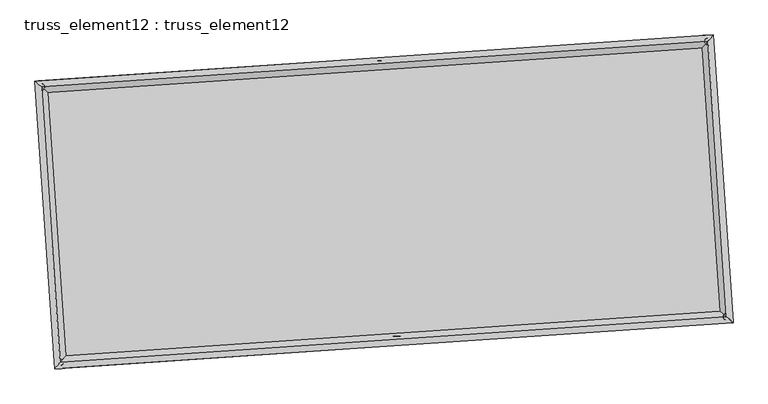
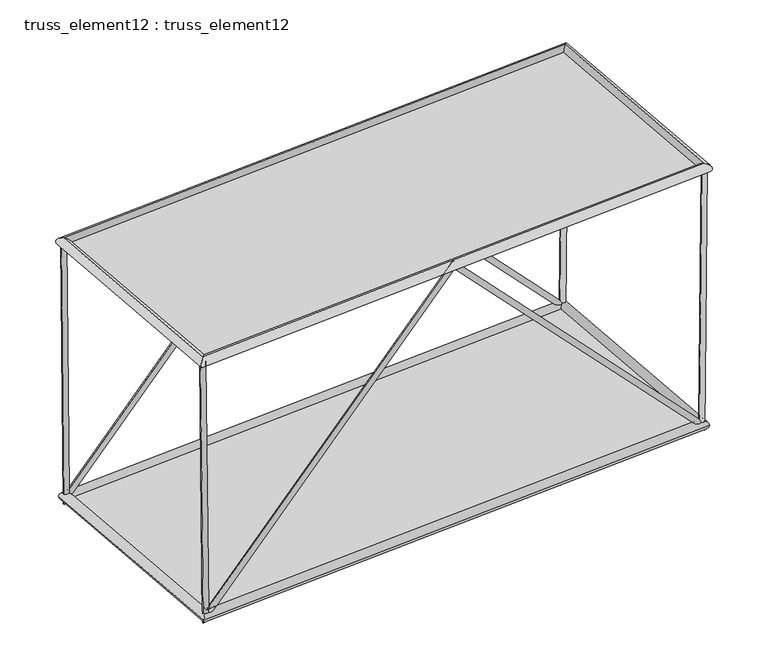
"""IFC4 building model written with IfcOpenShell, lengths in millimetres: plate geometry, truss_element12 : truss_element12."""

from ifc_helpers import new_model, si_unit, frame, origin, origin_with_axes, place, context, project, spatial, polyline, circle_curve, ellipse_curve, outline, extrude, source, transform, mapped, element, save
from ifc_brep_helpers import plane_surface, cylinder_surface, advanced_brep


def truss_element12_truss_element12_5452cb03(model_context):
    return source(origin(), model_context, "Body", "SolidModel", [
        advanced_brep(
        [(-3715.2018839, 2272.796917, 5000.248885), (-3814.3001969, 2259.4360138, 4999.2435881), (-3666.1746751, 2276.139896, 122.9048146), (-3762.8122077, 2262.9467841, -122.9048146), (1064.1683221, 2598.6840033, 5071.8637106), (1064.609821, 2592.1103415, 4927.6196838), (5793.6352732, 2921.1683763, 122.8985374), (5891.1257038, 2921.2121122, -122.8985374), (5843.5319155, 2924.5706386, 5000.2487185), (5943.5264514, 2924.78512, 4999.2255971)],
        [
            (0, 1, circle_curve(frame((-3764.7510404, 2266.1164654, 4999.7462366), z_axis=(-0.010051519791738989, -0.0006853749251947657, 0.9999492473176268), x_axis=(-0.1336091408985775, 0.991033882804214, -0.000663778839363479)), 50.0)),
            (1, 0, circle_curve(frame((-3764.7510404, 2266.1164654, 4999.7462366), z_axis=(-0.010051519791738989, -0.0006853749251947657, 0.9999492473176268), x_axis=(-0.1336091408985775, 0.991033882804214, -0.000663778839363479)), 50.0)),
            (0, 2),
            (2, 3, ellipse_curve(frame((-3714.4934414, 2269.54334, 0.0), z_axis=(-0.9276377400160163, -0.06325209121051249, 0.36808612613826514), x_axis=(0.3672334163736698, 0.025040250677613063, 0.9297916991157348)), 132.4731533, 50.0)),
            (3, 1),
            (3, 2, ellipse_curve(frame((-3714.4934414, 2269.54334, 0.0), z_axis=(-0.9276377400160163, -0.06325209121051249, 0.36808612613826514), x_axis=(0.3672334163736698, 0.025040250677613063, 0.9297916991157348)), 132.4731533, 50.0)),
            (2, 4),
            (4, 5, ellipse_curve(frame((1064.3890715, 2595.3971724, 4999.7416972), z_axis=(-0.9976833949926481, -0.06802823815490638, 4.657770887637942e-05), x_axis=(-4.6469806773262635e-05, -3.1685994756930008e-06, -0.9999999989152585)), 72.2790583, 50.0)),
            (5, 3),
            (5, 4, ellipse_curve(frame((1064.3890715, 2595.3971724, 4999.7416972), z_axis=(-0.9976833949926481, -0.06802823815490638, 4.657770887637942e-05), x_axis=(-4.6469806773262635e-05, -3.1685994756930008e-06, -0.9999999989152585)), 72.2790583, 50.0)),
            (4, 6),
            (6, 7, ellipse_curve(frame((5842.3804885, 2921.1902443, 0.0), z_axis=(-0.9276876380424469, -0.06325549356725449, -0.36795976513307666), x_axis=(-0.36710734809688195, -0.025031654561049187, 0.9298417130045366)), 132.4592623, 50.0)),
            (7, 5),
            (7, 6, ellipse_curve(frame((5842.3804885, 2921.1902443, 0.0), z_axis=(-0.9276876380424469, -0.06325549356725449, -0.36795976513307666), x_axis=(-0.36710734809688195, -0.025031654561049187, 0.9298417130045366)), 132.4592623, 50.0)),
            (8, 9, circle_curve(frame((5893.5291834, 2924.6778793, 4999.7371578), z_axis=(0.01022973898914847, 0.0006975270147915611, 0.9999474315664186), x_axis=(-0.0021518374254831385, 0.9999974566120504, -0.0006755480180010986)), 50.0)),
            (9, 8, circle_curve(frame((5893.5291834, 2924.6778793, 4999.7371578), z_axis=(0.01022973898914847, 0.0006975270147915611, 0.9999474315664186), x_axis=(-0.0021518374254831385, 0.9999974566120504, -0.0006755480180010986)), 50.0)),
            (6, 8),
            (9, 7),
        ],
        [
            plane_surface(frame((-3764.7510404, 2316.1164537, 4999.7805071), z_axis=(-0.010051519791740156, -0.0006853749251952957, 0.9999492473176268), x_axis=(0.9999494821989141, -6.889407663024368e-06, 0.010051517430706975))),
            cylinder_surface(frame((-3764.7510404, 2266.1164654, 4999.7462366), z_axis=(-0.010051519791738989, -0.0006853749251947657, 0.9999492473176268), x_axis=(-0.1336091408985775, 0.991033882804214, -0.000663778839363479)), 50.0),
            cylinder_surface(frame((-3714.4934414, 2269.54334, 0.0), z_axis=(-0.6901943166001666, -0.047061726774740055, -0.7220920988390671), x_axis=(-0.02041583735188898, 0.9987521038850324, -0.04557881712421584)), 50.0),
            cylinder_surface(frame((1064.3890715, 2595.3971724, 4999.7416972), z_axis=(-0.6901272026448988, -0.047057150529254216, 0.7221565403384463), x_axis=(-0.11534925749082463, 0.9922789548414734, -0.045574385075704216)), 50.0),
            plane_surface(frame((5893.5291834, 2874.6778915, 4999.772036), z_axis=(0.01022973898914786, 0.0006975270147901555, 0.9999474315664189), x_axis=(0.9999476748511464, -7.13589268563908e-06, -0.010229736500278365))),
            cylinder_surface(frame((5842.3804885, 2921.1902443, 0.0), z_axis=(-0.010229738989148472, -0.0006975270147915612, -0.9999474315664189), x_axis=(-0.0021518374254831385, 0.9999974566120504, -0.0006755480180010986)), 50.0),
        ],
        [
            (0, [[1, 2]]),
            (1, [[-1, 3, 4, 5]]),
            (1, [[-2, -5, 6, -3]]),
            (2, [[-4, 7, 8, 9]]),
            (2, [[-6, -9, 10, -7]]),
            (3, [[-8, 11, 12, 13]]),
            (3, [[-10, -13, 14, -11]]),
            (4, [[15, 16]]),
            (5, [[-12, 17, -16, 18]]),
            (5, [[-14, -18, -15, -17]]),
        ],
    ),
        advanced_brep(
        [(-3443.0889309, -1717.9366673, 5000.248885), (-3542.187244, -1731.2975705, 4999.2435881), (-3394.0617222, -1714.5936883, 122.9048146), (-3490.6992548, -1727.7868002, -122.9048146), (1336.281275, -1392.049581, 5071.8637106), (1336.7227739, -1398.6232428, 4927.6196838), (6065.7482261, -1069.565208, 122.8985374), (6163.2386567, -1069.5214721, -122.8985374), (6115.6448684, -1066.1629457, 5000.2487185), (6215.6394043, -1065.9484643, 4999.2255971)],
        [
            (0, 1, circle_curve(frame((-3492.6380875, -1724.6171189, 4999.7462366), z_axis=(-0.010051519791739193, -0.000685374925194784, 0.9999492473176267), x_axis=(-0.13360914089857726, 0.991033882804214, -0.0006637788393634854)), 50.0)),
            (1, 0, circle_curve(frame((-3492.6380875, -1724.6171189, 4999.7462366), z_axis=(-0.010051519791739193, -0.000685374925194784, 0.9999492473176267), x_axis=(-0.13360914089857726, 0.991033882804214, -0.0006637788393634854)), 50.0)),
            (0, 2),
            (2, 3, ellipse_curve(frame((-3442.3804885, -1721.1902443, 0.0), z_axis=(-0.9276377400160165, -0.06325209121051241, 0.3680861261382646), x_axis=(0.36723341637366924, 0.025040250677612983, 0.929791699115735)), 132.4731533, 50.0)),
            (3, 1),
            (3, 2, ellipse_curve(frame((-3442.3804885, -1721.1902443, 0.0), z_axis=(-0.9276377400160165, -0.06325209121051241, 0.3680861261382646), x_axis=(0.36723341637366924, 0.025040250677612983, 0.929791699115735)), 132.4731533, 50.0)),
            (2, 4),
            (4, 5, ellipse_curve(frame((1336.5020245, -1395.3364119, 4999.7416972), z_axis=(-0.9976833949926481, -0.0680282381549063, 4.657770887573745e-05), x_axis=(-4.646980677264766e-05, -3.168599475625738e-06, -0.9999999989152585)), 72.2790583, 50.0)),
            (5, 3),
            (5, 4, ellipse_curve(frame((1336.5020245, -1395.3364119, 4999.7416972), z_axis=(-0.9976833949926481, -0.0680282381549063, 4.657770887573745e-05), x_axis=(-4.646980677264766e-05, -3.168599475625738e-06, -0.9999999989152585)), 72.2790583, 50.0)),
            (4, 6),
            (6, 7, ellipse_curve(frame((6114.4934414, -1069.54334, 0.0), z_axis=(-0.9276876380424468, -0.06325549356725439, -0.36795976513307704), x_axis=(-0.3671073480968823, -0.025031654561049214, 0.9298417130045364)), 132.4592623, 50.0)),
            (7, 5),
            (7, 6, ellipse_curve(frame((6114.4934414, -1069.54334, 0.0), z_axis=(-0.9276876380424468, -0.06325549356725439, -0.36795976513307704), x_axis=(-0.3671073480968823, -0.025031654561049214, 0.9298417130045364)), 132.4592623, 50.0)),
            (8, 9, circle_curve(frame((6165.6421364, -1066.055705, 4999.7371578), z_axis=(0.010229738989148298, 0.0006975270147915052, 0.9999474315664186), x_axis=(-0.0021518374254831524, 0.9999974566120505, -0.0006755480180010431)), 50.0)),
            (9, 8, circle_curve(frame((6165.6421364, -1066.055705, 4999.7371578), z_axis=(0.010229738989148298, 0.0006975270147915052, 0.9999474315664186), x_axis=(-0.0021518374254831524, 0.9999974566120505, -0.0006755480180010431)), 50.0)),
            (6, 8),
            (9, 7),
        ],
        [
            plane_surface(frame((-3492.6380875, -1674.6171306, 4999.7805071), z_axis=(-0.010051519791740156, -0.0006853749251952938, 0.9999492473176268), x_axis=(0.9999494821989141, -6.889407663024368e-06, 0.010051517430706975))),
            cylinder_surface(frame((-3492.6380875, -1724.6171189, 4999.7462366), z_axis=(-0.010051519791739195, -0.0006853749251947842, 0.9999492473176269), x_axis=(-0.13360914089857726, 0.991033882804214, -0.0006637788393634854)), 50.0),
            cylinder_surface(frame((-3442.3804885, -1721.1902443, 0.0), z_axis=(-0.6901943166001662, -0.04706172677473995, -0.7220920988390676), x_axis=(-0.020415837351888903, 0.9987521038850324, -0.04557881712421575)), 50.0),
            cylinder_surface(frame((1336.5020245, -1395.3364119, 4999.7416972), z_axis=(-0.6901272026448991, -0.0470571505292542, 0.7221565403384458), x_axis=(-0.11534925749082446, 0.9922789548414734, -0.04557438507570417)), 50.0),
            plane_surface(frame((6165.6421364, -1116.0556928, 4999.772036), z_axis=(0.01022973898914786, 0.0006975270147901537, 0.9999474315664189), x_axis=(0.9999476748511464, -7.13589268563908e-06, -0.010229736500278365))),
            cylinder_surface(frame((6114.4934414, -1069.54334, 0.0), z_axis=(-0.0102297389891483, -0.0006975270147915053, -0.9999474315664189), x_axis=(-0.0021518374254831524, 0.9999974566120505, -0.0006755480180010431)), 50.0),
        ],
        [
            (0, [[1, 2]]),
            (1, [[-1, 3, 4, 5]]),
            (1, [[-2, -5, 6, -3]]),
            (2, [[-4, 7, 8, 9]]),
            (2, [[-6, -9, 10, -7]]),
            (3, [[-8, 11, 12, 13]]),
            (3, [[-10, -13, 14, -11]]),
            (4, [[15, 16]]),
            (5, [[-12, 17, -16, 18]]),
            (5, [[-14, -18, -15, -17]]),
        ],
    ),
        advanced_brep(
        [(-3492.6404759, -1724.619766, 4909.7462366), (-3492.635699, -1724.6144717, 5089.7462366), (-3764.7483147, 2266.114167, 5089.7462366), (-3764.753766, 2266.1187639, 4909.7462366), (5893.5269635, 2924.6752436, 5089.7371578), (5893.5314034, 2924.680515, 4909.7371579), (6165.6395791, -1066.053395, 5089.7371578), (6165.6446936, -1066.0580149, 4909.7371579)],
        [
            (0, 1, ellipse_curve(frame((-3492.6380875, -1724.6171189, 4999.7462366), z_axis=(-0.7535719234051445, 0.6573654662781055, 6.63138572682771e-07), x_axis=(-0.657365466277774, -0.7535719234054339, 6.631385726828099e-07)), 127.2792206, 90.0)),
            (1, 2),
            (2, 3, ellipse_curve(frame((-3764.7510404, 2266.1164654, 4999.7462366), z_axis=(-0.6573654662777743, -0.7535719234054338, 6.631385726828458e-07), x_axis=(0.7535719234051448, -0.6573654662781053, -6.631385726828071e-07)), 127.2792206, 90.0)),
            (3, 0),
            (1, 0, ellipse_curve(frame((-3492.6380875, -1724.6171189, 4999.7462366), z_axis=(-0.7535719234051445, 0.6573654662781055, 6.63138572682771e-07), x_axis=(-0.657365466277774, -0.7535719234054339, 6.631385726828099e-07)), 127.2792206, 90.0)),
            (3, 2, ellipse_curve(frame((-3764.7510404, 2266.1164654, 4999.7462366), z_axis=(-0.6573654662777743, -0.7535719234054338, 6.631385726828458e-07), x_axis=(0.7535719234051448, -0.6573654662781053, -6.631385726828071e-07)), 127.2792206, 90.0)),
            (2, 4),
            (4, 5, ellipse_curve(frame((5893.5291834, 2924.6778793, 4999.7371578), z_axis=(-0.7535719234051445, 0.6573654662781058, 6.63138572682843e-07), x_axis=(-0.6573654662777743, -0.7535719234054337, 6.631385726828096e-07)), 127.2792206, 90.0)),
            (5, 3),
            (5, 4, ellipse_curve(frame((5893.5291834, 2924.6778793, 4999.7371578), z_axis=(-0.7535719234051445, 0.6573654662781058, 6.63138572682843e-07), x_axis=(-0.6573654662777743, -0.7535719234054337, 6.631385726828096e-07)), 127.2792206, 90.0)),
            (4, 6),
            (6, 7, ellipse_curve(frame((6165.6421364, -1066.055705, 4999.7371578), z_axis=(0.6573654662777743, 0.7535719234054338, -6.631385726827738e-07), x_axis=(-0.7535719234051447, 0.6573654662781053, 6.631385726828074e-07)), 127.2792206, 90.0)),
            (7, 5),
            (7, 6, ellipse_curve(frame((6165.6421364, -1066.055705, 4999.7371578), z_axis=(0.6573654662777743, 0.7535719234054338, -6.631385726827738e-07), x_axis=(-0.7535719234051447, 0.6573654662781053, 6.631385726828074e-07)), 127.2792206, 90.0)),
            (6, 1),
            (0, 7),
        ],
        [
            cylinder_surface(frame((-3492.6380875, -1724.6171189, 4999.7462366), z_axis=(0.06802823822869596, -0.997683396074877, 0.0), x_axis=(-0.9976833956703363, -0.06802823820111187, 2.847736223492992e-05)), 90.0),
            cylinder_surface(frame((-3764.7510404, 2266.1164654, 4999.7462366), z_axis=(-0.9976833960744381, -0.06802823822866694, 9.378195632207894e-07), x_axis=(-0.06802823817713236, 0.9976833956982991, 2.753954267206479e-05)), 90.0),
            cylinder_surface(frame((5893.5291834, 2924.6778793, 4999.7371578), z_axis=(-0.06802823822869598, 0.9976833960748771, 0.0), x_axis=(0.9976833957218709, 0.06802823820462583, 2.6601723109199666e-05)), 90.0),
            cylinder_surface(frame((6165.6421364, -1066.055705, 4999.7371578), z_axis=(0.9976833960744381, 0.06802823822866695, -9.378195632207388e-07), x_axis=(0.06802823822866695, -0.9976833956947851, 2.75395426720648e-05)), 90.0),
        ],
        [
            (0, [[1, 2, 3, 4]]),
            (0, [[5, -4, 6, -2]]),
            (1, [[-3, 7, 8, 9]]),
            (1, [[-6, -9, 10, -7]]),
            (2, [[-8, 11, 12, 13]]),
            (2, [[-10, -13, 14, -11]]),
            (3, [[-12, 15, -1, 16]]),
            (3, [[-14, -16, -5, -15]]),
        ],
    ),
        advanced_brep(
        [(-3358.7115243, -1625.2761972, 0.0), (-3526.0494527, -1817.1042913, 0.0), (-3810.4074885, 2353.2123043, 0.0), (-3618.5793943, 2185.8743758, 0.0), (5926.0494527, 3017.1042913, 0.0), (5758.7115243, 2825.2761972, 0.0), (6210.4074885, -1153.2123043, 0.0), (6018.5793943, -985.8743758, 0.0)],
        [
            (0, 1, ellipse_curve(frame((-3442.3804885, -1721.1902443, 0.0), z_axis=(-0.7535719234054564, 0.6573654662780827, 0.0), x_axis=(-0.6573654662780827, -0.7535719234054563, 0.0)), 127.2792206, 90.0)),
            (1, 2),
            (2, 3, ellipse_curve(frame((-3714.4934414, 2269.54334, 0.0), z_axis=(-0.6573654662780827, -0.7535719234054565, 0.0), x_axis=(0.7535719234054565, -0.6573654662780822, 0.0)), 127.2792206, 90.0)),
            (3, 0),
            (1, 0, ellipse_curve(frame((-3442.3804885, -1721.1902443, 0.0), z_axis=(-0.7535719234054564, 0.6573654662780827, 0.0), x_axis=(-0.6573654662780827, -0.7535719234054563, 0.0)), 127.2792206, 90.0)),
            (3, 2, ellipse_curve(frame((-3714.4934414, 2269.54334, 0.0), z_axis=(-0.6573654662780827, -0.7535719234054565, 0.0), x_axis=(0.7535719234054565, -0.6573654662780822, 0.0)), 127.2792206, 90.0)),
            (2, 4),
            (4, 5, ellipse_curve(frame((5842.3804885, 2921.1902443, 0.0), z_axis=(-0.7535719234054563, 0.6573654662780826, 0.0), x_axis=(-0.6573654662780828, -0.7535719234054562, 0.0)), 127.2792206, 90.0)),
            (5, 3),
            (5, 4, ellipse_curve(frame((5842.3804885, 2921.1902443, 0.0), z_axis=(-0.7535719234054563, 0.6573654662780826, 0.0), x_axis=(-0.6573654662780828, -0.7535719234054562, 0.0)), 127.2792206, 90.0)),
            (4, 6),
            (6, 7, ellipse_curve(frame((6114.4934414, -1069.54334, 0.0), z_axis=(0.6573654662780825, 0.7535719234054565, 0.0), x_axis=(-0.7535719234054565, 0.6573654662780823, 0.0)), 127.2792206, 90.0)),
            (7, 5),
            (7, 6, ellipse_curve(frame((6114.4934414, -1069.54334, 0.0), z_axis=(0.6573654662780825, 0.7535719234054565, 0.0), x_axis=(-0.7535719234054565, 0.6573654662780823, 0.0)), 127.2792206, 90.0)),
            (6, 1),
            (0, 7),
        ],
        [
            cylinder_surface(frame((-3442.3804885, -1721.1902443, 0.0), z_axis=(0.06802823822869844, -0.9976833960748768, 0.0), x_axis=(-0.9976833960748768, -0.06802823822869844, 0.0)), 90.0),
            cylinder_surface(frame((-3714.4934414, 2269.54334, 0.0), z_axis=(-0.9976833960748768, -0.06802823822869929, 0.0), x_axis=(-0.06802823822869929, 0.9976833960748768, 0.0)), 90.0),
            cylinder_surface(frame((5842.3804885, 2921.1902443, 0.0), z_axis=(-0.06802823822869851, 0.9976833960748768, 0.0), x_axis=(0.9976833960748768, 0.06802823822869851, 0.0)), 90.0),
            cylinder_surface(frame((6114.4934414, -1069.54334, 0.0), z_axis=(0.9976833960748768, 0.06802823822869936, 0.0), x_axis=(0.06802823822869936, -0.9976833960748768, 0.0)), 90.0),
        ],
        [
            (0, [[1, 2, 3, 4]]),
            (0, [[5, -4, 6, -2]]),
            (1, [[-3, 7, 8, 9]]),
            (1, [[-6, -9, 10, -7]]),
            (2, [[-8, 11, 12, 13]]),
            (2, [[-10, -13, 14, -11]]),
            (3, [[-12, 15, -1, 16]]),
            (3, [[-14, -16, -5, -15]]),
        ],
    ),
        extrude(outline(polyline([(-3442.3804885, -1721.1902443), (-3714.4934414, 2269.54334), (5842.3804885, 2921.1902443), (6114.4934414, -1069.54334), (-3442.3804885, -1721.1902443)])), origin_with_axes(), (0.0, 0.0, 1.0), 20.0),
        extrude(outline(polyline([(-2000.0, 4840.3532934), (2000.0, 4840.3532934), (2000.0, -4840.3532933), (-2000.0, -4840.3532934), (-2000.0, 4840.3532934)])), frame((1200.445548, 600.0303802, 4999.7416972), z_axis=(9.356470067395495e-07, 6.37982126623162e-08, 0.9999999999995604), x_axis=(-0.06802823822869858, 0.9976833960748768, 0.0)), (0.0, 0.0, 1.0), 20.0),
    ])


if __name__ == "__main__":
    model = new_model("IFC4")
    model_context = context("Model", 3, world=origin())
    ifc_project = project(units=[si_unit("LENGTHUNIT", "METRE", prefix="MILLI")], contexts=[model_context])
    site = spatial("IfcSite", under=ifc_project)
    building = spatial("IfcBuilding", under=site)
    placement = place(None, origin())
    truss_element12_truss_element12_shape = truss_element12_truss_element12_5452cb03(model_context)
    element("IfcPlate", 1, ObjectType="truss_element12 : truss_element12", at=placement, inside=building, context=model_context, shape_type="MappedRepresentation", body=[
        mapped(truss_element12_truss_element12_shape, transform((0.0, 0.0, 0.0), x_axis=(1.0, 0.0, 0.0), y_axis=(0.0, 1.0, 0.0), z_axis=(0.0, 0.0, 1.0))),
    ])
    save(model, "model.ifc")

# Revit data of these elements
# Type "truss_element12 : truss_element12"
#   steellbar1 = 90 mm
#   steelbar2 = 50 mm
#   offset1 = 5000 mm
#   M = Default Roof
# Element 1 (IfcPlate, "truss_element12 : truss_element12")
#   Materials on its faces: "Default Roof"
# Materials
#   "Default Roof": class "Miscellaneous", colour RGB 0 127 0, transparency 0, Comments = "Rendering appearance not upgraded Rendering appearance not upgraded ", Cost = 0
